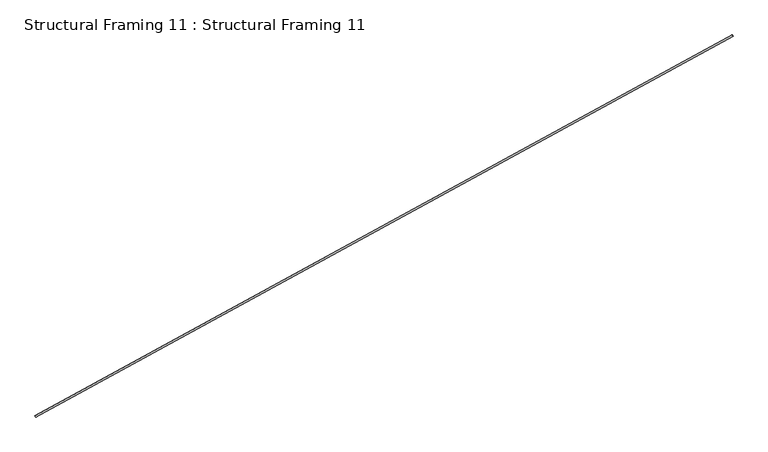
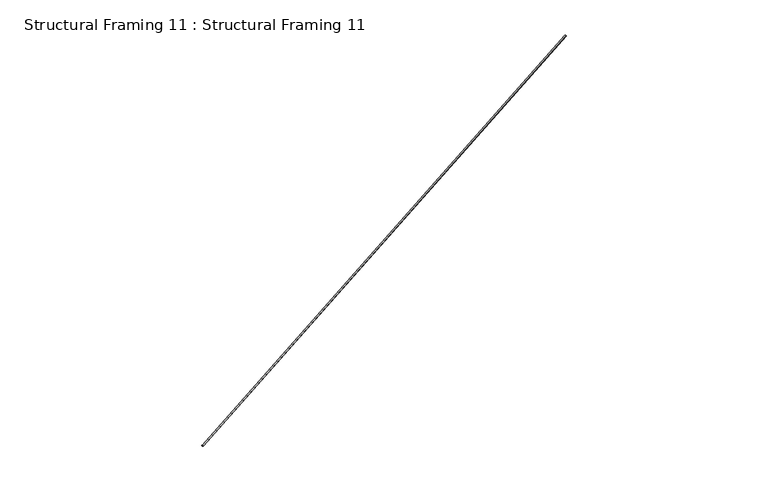
"""IFC4 building model written with IfcOpenShell, lengths in millimetres: beam geometry, Structural Framing 11 : Structural Framing 11."""

import ifcopenshell
import ifcopenshell.guid

model = None  # the IFC model being written
_history = None  # IfcOwnerHistory: only IFC2X3 demands one
_inside = {}  # id of a spatial element -> (the spatial element, [elements in it])
_under = {}  # id of a project, library or spatial element -> (it, [spatial elements below it])
_declared = {}  # id of a project -> (the project, [libraries it declares])
_typed = {}  # id of a type object -> (the type object, [elements of that type])
_made_of = {}  # id of a material, layer set ... -> (it, [elements and type objects made of it])


def new_model(schema):
    """Start an empty IFC model of exactly this schema.

    Asked for "IFC4X3", IfcOpenShell would pick the latest addendum, in which some entities
    have other attributes; the version numbers below select the first issue.
    IFC2X3 requires an IfcOwnerHistory on every rooted entity: one is made here for all.
    """
    global model, _history
    if schema == "IFC4X3":
        model = ifcopenshell.file(schema_version=(4, 3, 0, 0))
    else:
        model = ifcopenshell.file(schema=schema)
    _inside.clear()
    _under.clear()
    _declared.clear()
    _typed.clear()
    _made_of.clear()
    _history = None
    if model.schema == "IFC2X3":
        org = make("IfcOrganization", Name="unknown")
        user = make(
            "IfcPersonAndOrganization",
            ThePerson=make("IfcPerson", FamilyName="unknown"),
            TheOrganization=org,
        )
        app = make(
            "IfcApplication",
            ApplicationDeveloper=org,
            Version="unknown",
            ApplicationFullName="unknown",
            ApplicationIdentifier="unknown",
        )
        _history = make(
            "IfcOwnerHistory",
            OwningUser=user,
            OwningApplication=app,
            ChangeAction="ADDED",
            CreationDate=0,
        )
    return model


def make(cls, **values):
    """One entity of the class cls with the attributes given. An attribute that is None is left unset."""
    return model.create_entity(
        cls, **{name: value for name, value in values.items() if value is not None}
    )


def rooted(cls, **values):
    """An entity with a GlobalId (a new one), such as an element, a storey or a relation."""
    return make(cls, GlobalId=ifcopenshell.guid.new(), OwnerHistory=_history, **values)


def si_unit(unit_type, name, prefix=None):
    """IfcSIUnit, for example si_unit("LENGTHUNIT", "METRE", prefix="MILLI")."""
    return make("IfcSIUnit", UnitType=unit_type, Prefix=prefix, Name=name)


def assignment(units):
    """IfcUnitAssignment: the units of a project."""
    return None if units is None else make("IfcUnitAssignment", Units=units)


def point(xyz):
    """IfcCartesianPoint."""
    return None if xyz is None else make("IfcCartesianPoint", Coordinates=xyz)


def direction(xyz):
    """IfcDirection."""
    return None if xyz is None else make("IfcDirection", DirectionRatios=xyz)


def frame(location, z_axis=None, x_axis=None):
    """IfcAxis2Placement3D, a coordinate frame: its origin and axes. An axis left out is left unset."""
    return make(
        "IfcAxis2Placement3D",
        Location=point(location),
        Axis=direction(z_axis),
        RefDirection=direction(x_axis),
    )


def frame_2d(location, x_axis=None):
    """IfcAxis2Placement2D, a coordinate frame in the plane: its origin and x axis."""
    return make(
        "IfcAxis2Placement2D", Location=point(location), RefDirection=direction(x_axis)
    )


def origin():
    """The frame at (0, 0, 0) with its axes left unset."""
    return frame((0.0, 0.0, 0.0))


def origin_2d():
    """The frame at (0, 0) in the plane with its x axis left unset."""
    return frame_2d((0.0, 0.0))


def place(relative_to, where):
    """IfcLocalPlacement: puts the frame where relative to a parent placement (None: the world)."""
    return make(
        "IfcLocalPlacement", PlacementRelTo=relative_to, RelativePlacement=where
    )


def context(
    kind, dimensions, precision=None, world=None, true_north=None, identifier=None
):
    """IfcGeometricRepresentationContext, for example the 3D "Model" context."""
    return make(
        "IfcGeometricRepresentationContext",
        ContextIdentifier=identifier,
        ContextType=kind,
        CoordinateSpaceDimension=dimensions,
        Precision=precision,
        WorldCoordinateSystem=world,
        TrueNorth=true_north,
    )


def project(units=None, contexts=None):
    """IfcProject with its units and contexts."""
    return rooted(
        "IfcProject",
        Name="project",
        RepresentationContexts=contexts,
        UnitsInContext=assignment(units),
    )


def spatial(cls, under=None, at=None, **own):
    """A site, building, storey or space (cls), placed at a placement, below another one or the project."""
    s = rooted(cls, ObjectPlacement=at, **own)
    if under is not None:
        _under.setdefault(under.id(), (under, []))[1].append(s)
    return s


def circle_curve(where, radius):
    """IfcCircle in the frame where."""
    return make("IfcCircle", Position=where, Radius=radius)


def trimmed(basis, trim1, trim2, sense, master):
    """IfcTrimmedCurve: the piece of a basis curve between two trims."""
    return make(
        "IfcTrimmedCurve",
        BasisCurve=basis,
        Trim1=trim1,
        Trim2=trim2,
        SenseAgreement=sense,
        MasterRepresentation=master,
    )


def segment(curve, same_sense, transition):
    """IfcCompositeCurveSegment."""
    return make(
        "IfcCompositeCurveSegment",
        Transition=transition,
        SameSense=same_sense,
        ParentCurve=curve,
    )


def composite_curve(segments, self_intersect=None):
    """IfcCompositeCurve: segments joined end to end."""
    return make("IfcCompositeCurve", Segments=segments, SelfIntersect=self_intersect)


def outline(outer, holes=None, kind="AREA"):
    """IfcArbitraryClosedProfileDef: a profile drawn as a closed curve; with holes, ...WithVoids."""
    if holes is None:
        return make("IfcArbitraryClosedProfileDef", ProfileType=kind, OuterCurve=outer)
    return make(
        "IfcArbitraryProfileDefWithVoids",
        ProfileType=kind,
        OuterCurve=outer,
        InnerCurves=holes,
    )


def extrude(swept, where, along, depth):
    """IfcExtrudedAreaSolid: the profile swept, set in the frame where, extruded along a direction by depth."""
    return make(
        "IfcExtrudedAreaSolid",
        SweptArea=swept,
        Position=where,
        ExtrudedDirection=direction(along),
        Depth=depth,
    )


def shape(context_of_items, identifier, shape_type, items):
    """IfcShapeRepresentation: the items that make up one representation, for example the "Body"."""
    return make(
        "IfcShapeRepresentation",
        ContextOfItems=context_of_items,
        RepresentationIdentifier=identifier,
        RepresentationType=shape_type,
        Items=items,
    )


def source(mapping_origin, context_of_items, identifier, shape_type, items):
    """IfcRepresentationMap: a shape defined once, which mapped items show again and again."""
    return make(
        "IfcRepresentationMap",
        MappingOrigin=mapping_origin,
        MappedRepresentation=shape(context_of_items, identifier, shape_type, items),
    )


def transform(
    local_origin,
    x_axis=None,
    y_axis=None,
    z_axis=None,
    scale=None,
    scale2=None,
    scale3=None,
    uniform=True,
):
    """IfcCartesianTransformationOperator3D, or its non-uniform kind. x_axis, y_axis, z_axis: its Axis1, 2, 3."""
    if uniform:
        return make(
            "IfcCartesianTransformationOperator3D",
            Axis1=direction(x_axis),
            Axis2=direction(y_axis),
            LocalOrigin=point(local_origin),
            Scale=scale,
            Axis3=direction(z_axis),
        )
    return make(
        "IfcCartesianTransformationOperator3DnonUniform",
        Axis1=direction(x_axis),
        Axis2=direction(y_axis),
        LocalOrigin=point(local_origin),
        Scale=scale,
        Axis3=direction(z_axis),
        Scale2=scale2,
        Scale3=scale3,
    )


def mapped(mapping_source, mapping_target):
    """IfcMappedItem: shows the shape of a source again, moved by a transform."""
    return make(
        "IfcMappedItem", MappingSource=mapping_source, MappingTarget=mapping_target
    )


def made_of(thing, what):
    """Note that an element or type object is made of a material, layer set ...; save() writes the relation."""
    if what is not None:
        _made_of.setdefault(what.id(), (what, []))[1].append(thing)
    return thing


def element(
    cls,
    number,
    at=None,
    inside=None,
    cuts=None,
    type_object=None,
    material=None,
    context=None,
    identifier="Body",
    shape_type=None,
    held_by="IfcProductDefinitionShape",
    body=None,
    shapes=None,
    **own,
):
    """One element of the class cls, such as IfcWall. Its Tag is "e" and its number.

    at: its placement. inside: the storey or other place that contains it. cuts: it is an
    opening in that element (IfcRelVoidsElement). A single representation is given by context,
    identifier, shape_type and body (its items); several are given by shapes. held_by: the class
    of the entity that holds the representations. save() writes the other relations.
    """
    e = rooted(cls, Tag="e%d" % number, ObjectPlacement=at, **own)
    if body is not None:
        shapes = [shape(context, identifier, shape_type, body)]
    if shapes is not None:
        e.Representation = make(held_by, Representations=shapes)
    if inside is not None:
        _inside.setdefault(inside.id(), (inside, []))[1].append(e)
    if cuts is not None:
        rooted(
            "IfcRelVoidsElement", RelatingBuildingElement=cuts, RelatedOpeningElement=e
        )
    if type_object is not None:
        _typed.setdefault(type_object.id(), (type_object, []))[1].append(e)
    return made_of(e, material)


def aggregate(whole, parts):
    """IfcRelAggregates: a whole, such as a stair, and the parts it consists of."""
    return rooted("IfcRelAggregates", RelatingObject=whole, RelatedObjects=parts)


def save(model, path):
    """Write the relations noted so far, then the file.

    IfcRelAggregates (storeys below a building ...), IfcRelContainedInSpatialStructure (elements
    in a storey), IfcRelDefinesByType, IfcRelAssociatesMaterial and IfcRelDeclares: one each for
    every whole, place, type object, material and project.
    """
    for whole, parts in _under.values():
        aggregate(whole, parts)
    for where, things in _inside.values():
        rooted(
            "IfcRelContainedInSpatialStructure",
            RelatedElements=things,
            RelatingStructure=where,
        )
    for kind, things in _typed.values():
        rooted("IfcRelDefinesByType", RelatedObjects=things, RelatingType=kind)
    for what, things in _made_of.values():
        rooted("IfcRelAssociatesMaterial", RelatedObjects=things, RelatingMaterial=what)
    for by, libraries in _declared.values():
        rooted("IfcRelDeclares", RelatingContext=by, RelatedDefinitions=libraries)
    model.write(path)


def structural_framing_11_structural_framing_11_4b418407(model_context):
    return source(origin(), model_context, "Body", "SweptSolid", [
        extrude(outline(composite_curve([segment(trimmed(circle_curve(origin_2d(), 6.35), [point((0.0, 6.3499999))], [point((0.0, -6.35))], False, "CARTESIAN"), True, "CONTINUOUS"), segment(trimmed(circle_curve(origin_2d(), 6.35), [point((0.0, -6.35))], [point((0.0, 6.3499999))], False, "CARTESIAN"), True, "CONTINUOUS")], self_intersect=False)), frame((12605.5334333, 4177.5989868, 4934.3713104), z_axis=(0.8714985593718706, 0.47575600371495885, 0.11893900092873712), x_axis=(0.0, -0.24253562503632659, 0.9701425001453335)), (0.0, 0.0, 1.0), 6120.4961437),
    ])


if __name__ == "__main__":
    model = new_model("IFC4")
    model_context = context("Model", 3, world=origin())
    ifc_project = project(units=[si_unit("LENGTHUNIT", "METRE", prefix="MILLI")], contexts=[model_context])
    site = spatial("IfcSite", under=ifc_project)
    building = spatial("IfcBuilding", under=site)
    placement = place(None, origin())
    structural_framing_11_structural_framing_11_shape = structural_framing_11_structural_framing_11_4b418407(model_context)
    element("IfcBeam", 1, ObjectType="Structural Framing 11 : Structural Framing 11", at=placement, inside=building, context=model_context, shape_type="MappedRepresentation", body=[
        mapped(structural_framing_11_structural_framing_11_shape, transform((0.0, 0.0, 0.0), x_axis=(1.0, 0.0, 0.0), y_axis=(0.0, 1.0, 0.0), z_axis=(0.0, 0.0, 1.0))),
    ])
    save(model, "model.ifc")

# Revit data of these elements
# Type "Structural Framing 11 : Structural Framing 11"
#   Structural Material [instance default] = EXISTING LATERAL BRACING (1/4" CABLE)
# Element 1 (IfcBeam, "Structural Framing 11 : Structural Framing 11")
#   Materials on its faces: "EXISTING LATERAL BRACING (1/4\" CABLE)"
# Materials
#   "EXISTING LATERAL BRACING (1/4\" CABLE)": class "Generic", colour RGB 120 120 120, transparency 0, Cost = 0
